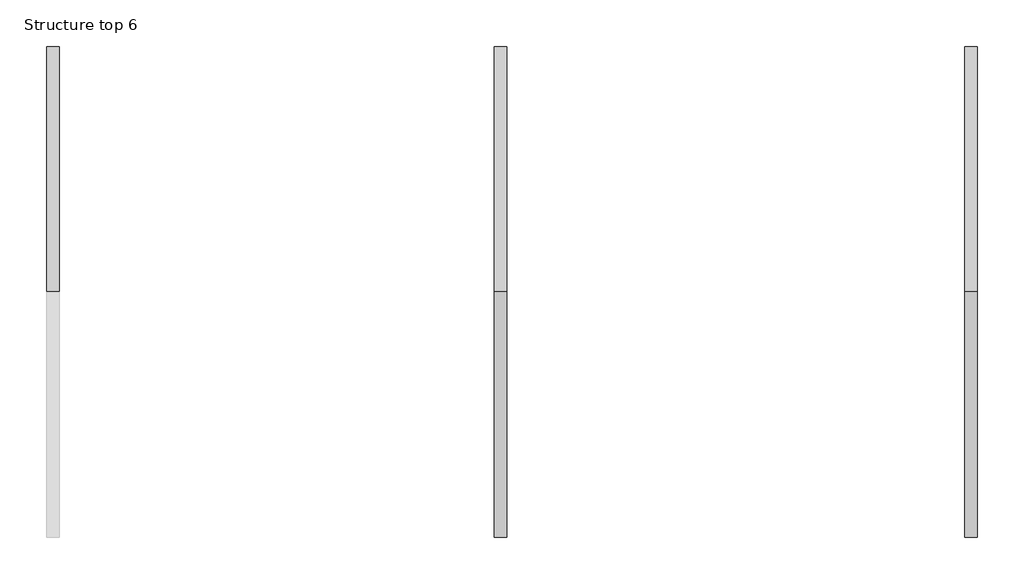
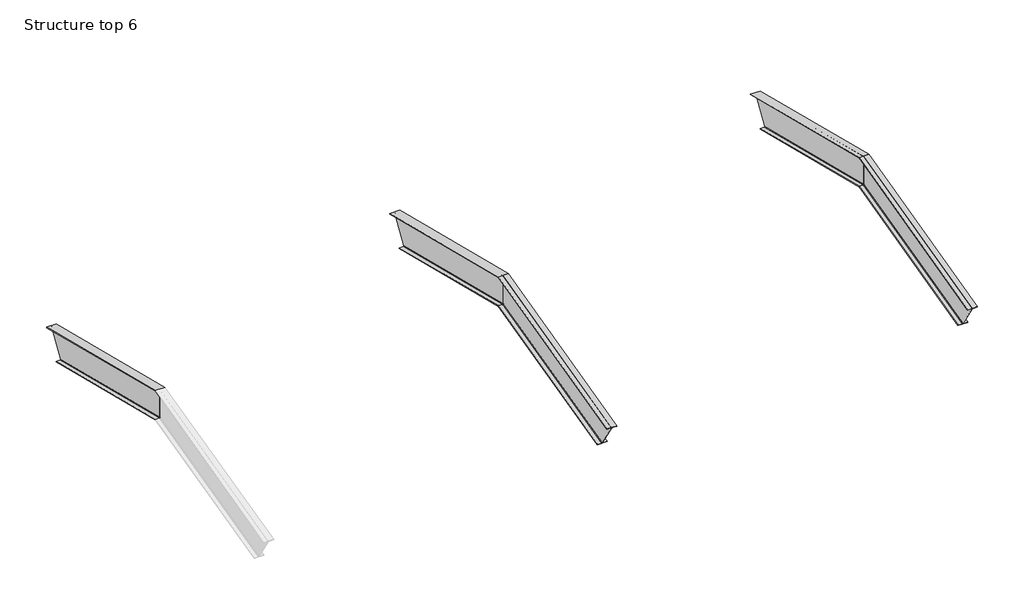
# One storey, part 2 of 2: 5 beams.
"""IFC4 building model written with IfcOpenShell, lengths in millimetres."""

from ifc_helpers import new_model, si_unit, frame, origin, place, context, project, spatial, polyline, ellipse_curve, element, save
from ifc_brep_helpers import plane_surface, revolved_surface, advanced_brep

model = new_model("IFC4")

# Units and contexts
model_context = context("Model", 3, world=origin())
ifc_project = project(units=[si_unit("LENGTHUNIT", "METRE", prefix="MILLI")], contexts=[model_context])

# Site, building, storey
site = spatial("IfcSite", under=ifc_project)
building = spatial("IfcBuilding", under=site)
storey = spatial("IfcBuildingStorey", under=building, Name="Structure top 6", Elevation=5867.6650904)

# Beams
placement = place(None, origin())
element("IfcBeam", 1, ObjectType="W Shapes : W 6X18.5", at=placement, inside=storey, context=model_context, shape_type="AdvancedBrep", body=[
    advanced_brep(
    [(17988.1744333, 7113.772024, 5183.7974927), (18053.8334333, 7113.772024, 5183.7974927), (18053.8334333, 9790.156119, 4514.7014689), (17988.1744333, 9790.156119, 4514.7014689), (17980.5544333, 7113.772024, 5191.6520089), (17980.5544333, 9794.417492, 4521.4906419), (17980.5544333, 7113.772024, 5640.4067021), (17980.5544333, 10037.8839324, 4909.378725), (17988.1744333, 7113.772024, 5648.2612183), (17988.1744333, 10042.1453053, 4916.1678979), (18053.8334333, 7113.772024, 5648.2612183), (18053.8334333, 10042.1453053, 4916.1678979), (18053.8334333, 7113.772024, 5658.2102722), (18053.8334333, 10047.5430444, 4924.7675171), (17901.4334333, 7113.772024, 5658.2102722), (17901.4334333, 10047.5430444, 4924.7675171), (17901.4334333, 7113.772024, 5648.2612183), (17901.4334333, 10042.1453053, 4916.1678979), (17967.0924333, 7113.772024, 5648.2612183), (17967.0924333, 10042.1453053, 4916.1678979), (17974.7124333, 7113.772024, 5640.4067021), (17974.7124333, 10037.8839324, 4909.378725), (17974.7124333, 7113.772024, 5191.6520089), (17974.7124333, 9794.417492, 4521.4906419), (17967.0924333, 7113.772024, 5183.7974927), (17967.0924333, 9790.156119, 4514.7014689), (17901.4334333, 7113.772024, 5183.7974927), (17901.4334333, 9790.156119, 4514.7014689), (17901.4334333, 7113.772024, 5173.8484388), (17901.4334333, 9784.75838, 4506.1018498), (18053.8334333, 7113.772024, 5173.8484388), (18053.8334333, 9784.75838, 4506.1018498)],
    [
        (0, 1),
        (1, 2),
        (2, 3),
        (3, 0),
        (4, 0, ellipse_curve(frame((17988.1744333, 7113.772024, 5191.6520089), z_axis=(0.0, -1.0, 0.0), x_axis=(0.0, 0.0, -1.0)), 7.8545162, 7.62)),
        (3, 5, ellipse_curve(frame((17988.1744333, 9794.417492, 4521.4906419), z_axis=(0.0, 0.8469796531886612, -0.5316253070390979), x_axis=(0.0, 0.5316253070390978, 0.8469796531886611)), 8.0157451, 7.62)),
        (5, 4),
        (6, 4),
        (5, 7),
        (7, 6),
        (8, 6, ellipse_curve(frame((17988.1744333, 7113.772024, 5640.4067021), z_axis=(0.0, -1.0, 0.0), x_axis=(0.0, 0.0, -1.0)), 7.8545162, 7.62)),
        (7, 9, ellipse_curve(frame((17988.1744333, 10037.8839324, 4909.378725), z_axis=(0.0, 0.8469796531886612, -0.5316253070390979), x_axis=(0.0, 0.5316253070390978, 0.8469796531886611)), 8.0157451, 7.62)),
        (9, 8),
        (10, 8),
        (9, 11),
        (11, 10),
        (12, 10),
        (11, 13),
        (13, 12),
        (14, 12),
        (13, 15),
        (15, 14),
        (16, 14),
        (15, 17),
        (17, 16),
        (18, 16),
        (17, 19),
        (19, 18),
        (20, 18, ellipse_curve(frame((17967.0924333, 7113.772024, 5640.4067021), z_axis=(0.0, -1.0, 0.0), x_axis=(0.0, 0.0, -1.0)), 7.8545162, 7.62)),
        (19, 21, ellipse_curve(frame((17967.0924333, 10037.8839324, 4909.378725), z_axis=(0.0, 0.8469796531886612, -0.5316253070390979), x_axis=(0.0, 0.5316253070390978, 0.8469796531886611)), 8.0157451, 7.62)),
        (21, 20),
        (22, 20),
        (21, 23),
        (23, 22),
        (24, 22, ellipse_curve(frame((17967.0924333, 7113.772024, 5191.6520089), z_axis=(0.0, -1.0, 0.0), x_axis=(0.0, 0.0, -1.0)), 7.8545162, 7.62)),
        (23, 25, ellipse_curve(frame((17967.0924333, 9794.417492, 4521.4906419), z_axis=(0.0, 0.8469796531886612, -0.5316253070390979), x_axis=(0.0, 0.5316253070390978, 0.8469796531886611)), 8.0157451, 7.62)),
        (25, 24),
        (26, 24),
        (25, 27),
        (27, 26),
        (28, 26),
        (27, 29),
        (29, 28),
        (30, 28),
        (29, 31),
        (31, 30),
        (1, 30),
        (31, 2),
    ],
    [
        plane_surface(frame((18053.8334333, 7002.1447176, 5211.7043193), z_axis=(0.0, 0.24253562503633308, 0.9701425001453319), x_axis=(0.0, 0.9701425001453319, -0.24253562503633308))),
        revolved_surface(polyline([(17980.5544333, 9796.830743469387, 4520.887328982653), (17980.5544333, 7111.923902529412, 5192.114039217647)]), (17988.1744333, 7003.992839, 5219.0968051), (0.0, 0.9701425001453319, -0.24253562503633308)),
        plane_surface(frame((17980.5544333, 7003.992839, 5219.0968051), z_axis=(1.0, 0.0, 0.0), x_axis=(0.0, 0.9701425001453319, -0.24253562503633308))),
        revolved_surface(polyline([(17980.5544333, 10040.297183869387, 4908.775412082653), (17980.5544333, 7111.923902529412, 5640.868732417647)]), (17988.1744333, 7109.5821786, 5641.4541634), (0.0, 0.9701425001453319, -0.24253562503633308)),
        plane_surface(frame((17988.1744333, 7111.4303001, 5648.8466493), z_axis=(0.0, -0.24253562503633308, -0.9701425001453319), x_axis=(0.0, 0.9701425001453319, -0.24253562503633308))),
        plane_surface(frame((18053.8334333, 7111.4303001, 5648.8466493), z_axis=(1.0, 0.0, 0.0), x_axis=(0.0, 0.9701425001453319, -0.24253562503633308))),
        plane_surface(frame((18053.8334333, 7113.7712539, 5658.2104647), z_axis=(0.0, 0.24253562503633308, 0.9701425001453319), x_axis=(0.0, 0.9701425001453319, -0.24253562503633308))),
        plane_surface(frame((17901.4334333, 7113.7712539, 5658.2104647), z_axis=(-1.0, 0.0, 0.0), x_axis=(0.0, 0.9701425001453319, -0.24253562503633308))),
        plane_surface(frame((17901.4334333, 7111.4303001, 5648.8466493), z_axis=(0.0, -0.24253562503633308, -0.9701425001453319), x_axis=(0.0, 0.9701425001453319, -0.24253562503633308))),
        revolved_surface(polyline([(17959.4724333, 10040.297183869387, 4908.775412082653), (17959.4724333, 7111.923902529412, 5640.868732417647)]), (17967.0924333, 7109.5821786, 5641.4541634), (0.0, 0.9701425001453319, -0.24253562503633308)),
        plane_surface(frame((17974.7124333, 7109.5821786, 5641.4541634), z_axis=(-1.0, 0.0, 0.0), x_axis=(0.0, 0.9701425001453319, -0.24253562503633308))),
        revolved_surface(polyline([(17959.4724333, 9796.830743469387, 4520.887328982653), (17959.4724333, 7111.923902529412, 5192.114039217647)]), (17967.0924333, 7003.992839, 5219.0968051), (0.0, 0.9701425001453319, -0.24253562503633308)),
        plane_surface(frame((17967.0924333, 7002.1447176, 5211.7043193), z_axis=(0.0, 0.24253562503633308, 0.9701425001453319), x_axis=(0.0, 0.9701425001453319, -0.24253562503633308))),
        plane_surface(frame((17901.4334333, 7002.1447176, 5211.7043193), z_axis=(-1.0, 0.0, 0.0), x_axis=(0.0, 0.9701425001453319, -0.24253562503633308))),
        plane_surface(frame((17901.4334333, 6999.8037637, 5202.3405039), z_axis=(0.0, -0.24253562503633308, -0.9701425001453319), x_axis=(0.0, 0.9701425001453319, -0.24253562503633308))),
        plane_surface(frame((18053.8334333, 6999.8037637, 5202.3405039), z_axis=(1.0, 0.0, 0.0), x_axis=(0.0, 0.9701425001453319, -0.24253562503633308))),
        plane_surface(frame((17977.6370052, 7113.772024, 5658.2135449), z_axis=(0.0, -1.0, 0.0), x_axis=(0.0, 0.0, 1.0))),
        plane_surface(frame((17977.6370052, 10047.54482, 4924.7703459), z_axis=(0.0, 0.8469796531886612, -0.5316253070390979), x_axis=(1.0, 0.0, 0.0))),
    ],
    [
        (0, [[1, 2, 3, 4]]),
        (1, [[5, -4, 6, 7]]),
        (2, [[8, -7, 9, 10]]),
        (3, [[11, -10, 12, 13]]),
        (4, [[14, -13, 15, 16]]),
        (5, [[17, -16, 18, 19]]),
        (6, [[20, -19, 21, 22]]),
        (7, [[23, -22, 24, 25]]),
        (8, [[26, -25, 27, 28]]),
        (9, [[29, -28, 30, 31]]),
        (10, [[32, -31, 33, 34]]),
        (11, [[35, -34, 36, 37]]),
        (12, [[38, -37, 39, 40]]),
        (13, [[41, -40, 42, 43]]),
        (14, [[44, -43, 45, 46]]),
        (15, [[47, -46, 48, -2]]),
        (16, [[-1, -5, -8, -11, -14, -17, -20, -23, -26, -29, -32, -35, -38, -41, -44, -47]]),
        (17, [[-48, -45, -42, -39, -36, -33, -30, -27, -24, -21, -18, -15, -12, -9, -6, -3]]),
    ],
),
])
element("IfcBeam", 2, ObjectType="W Shapes : W 6X18.5", at=placement, inside=storey, context=model_context, shape_type="AdvancedBrep", body=[
    advanced_brep(
    [(23341.2244333, 7113.772024, 5183.7974927), (23406.8834333, 7113.772024, 5183.7974927), (23406.8834333, 9790.156119, 4514.7014689), (23341.2244333, 9790.156119, 4514.7014689), (23333.6044333, 7113.772024, 5191.6520089), (23333.6044333, 9794.417492, 4521.4906419), (23333.6044333, 7113.772024, 5640.4067021), (23333.6044333, 10037.8839324, 4909.378725), (23341.2244333, 7113.772024, 5648.2612183), (23341.2244333, 10042.1453053, 4916.1678979), (23406.8834333, 7113.772024, 5648.2612183), (23406.8834333, 10042.1453053, 4916.1678979), (23406.8834333, 7113.772024, 5658.2102722), (23406.8834333, 10047.5430444, 4924.7675171), (23254.4834333, 7113.772024, 5658.2102722), (23254.4834333, 10047.5430444, 4924.7675171), (23254.4834333, 7113.772024, 5648.2612183), (23254.4834333, 10042.1453053, 4916.1678979), (23320.1424333, 7113.772024, 5648.2612183), (23320.1424333, 10042.1453053, 4916.1678979), (23327.7624333, 7113.772024, 5640.4067021), (23327.7624333, 10037.8839324, 4909.378725), (23327.7624333, 7113.772024, 5191.6520089), (23327.7624333, 9794.417492, 4521.4906419), (23320.1424333, 7113.772024, 5183.7974927), (23320.1424333, 9790.156119, 4514.7014689), (23254.4834333, 7113.772024, 5183.7974927), (23254.4834333, 9790.156119, 4514.7014689), (23254.4834333, 7113.772024, 5173.8484388), (23254.4834333, 9784.75838, 4506.1018498), (23406.8834333, 7113.772024, 5173.8484388), (23406.8834333, 9784.75838, 4506.1018498)],
    [
        (0, 1),
        (1, 2),
        (2, 3),
        (3, 0),
        (4, 0, ellipse_curve(frame((23341.2244333, 7113.772024, 5191.6520089), z_axis=(0.0, -1.0, 0.0), x_axis=(0.0, 0.0, -1.0)), 7.8545162, 7.62)),
        (3, 5, ellipse_curve(frame((23341.2244333, 9794.417492, 4521.4906419), z_axis=(0.0, 0.8469796531886612, -0.5316253070390979), x_axis=(0.0, 0.5316253070390978, 0.8469796531886611)), 8.0157451, 7.62)),
        (5, 4),
        (6, 4),
        (5, 7),
        (7, 6),
        (8, 6, ellipse_curve(frame((23341.2244333, 7113.772024, 5640.4067021), z_axis=(0.0, -1.0, 0.0), x_axis=(0.0, 0.0, -1.0)), 7.8545162, 7.62)),
        (7, 9, ellipse_curve(frame((23341.2244333, 10037.8839324, 4909.378725), z_axis=(0.0, 0.8469796531886612, -0.5316253070390979), x_axis=(0.0, 0.5316253070390978, 0.8469796531886611)), 8.0157451, 7.62)),
        (9, 8),
        (10, 8),
        (9, 11),
        (11, 10),
        (12, 10),
        (11, 13),
        (13, 12),
        (14, 12),
        (13, 15),
        (15, 14),
        (16, 14),
        (15, 17),
        (17, 16),
        (18, 16),
        (17, 19),
        (19, 18),
        (20, 18, ellipse_curve(frame((23320.1424333, 7113.772024, 5640.4067021), z_axis=(0.0, -1.0, 0.0), x_axis=(0.0, 0.0, -1.0)), 7.8545162, 7.62)),
        (19, 21, ellipse_curve(frame((23320.1424333, 10037.8839324, 4909.378725), z_axis=(0.0, 0.8469796531886612, -0.5316253070390979), x_axis=(0.0, 0.5316253070390978, 0.8469796531886611)), 8.0157451, 7.62)),
        (21, 20),
        (22, 20),
        (21, 23),
        (23, 22),
        (24, 22, ellipse_curve(frame((23320.1424333, 7113.772024, 5191.6520089), z_axis=(0.0, -1.0, 0.0), x_axis=(0.0, 0.0, -1.0)), 7.8545162, 7.62)),
        (23, 25, ellipse_curve(frame((23320.1424333, 9794.417492, 4521.4906419), z_axis=(0.0, 0.8469796531886612, -0.5316253070390979), x_axis=(0.0, 0.5316253070390978, 0.8469796531886611)), 8.0157451, 7.62)),
        (25, 24),
        (26, 24),
        (25, 27),
        (27, 26),
        (28, 26),
        (27, 29),
        (29, 28),
        (30, 28),
        (29, 31),
        (31, 30),
        (1, 30),
        (31, 2),
    ],
    [
        plane_surface(frame((23406.8834333, 7002.1447176, 5211.7043193), z_axis=(0.0, 0.24253562503633308, 0.9701425001453319), x_axis=(0.0, 0.9701425001453319, -0.24253562503633308))),
        revolved_surface(polyline([(23333.604433300003, 9796.830743469387, 4520.887328982653), (23333.604433300003, 7111.923902529412, 5192.114039217647)]), (23341.2244333, 7003.992839, 5219.0968051), (0.0, 0.9701425001453319, -0.24253562503633308)),
        plane_surface(frame((23333.6044333, 7003.992839, 5219.0968051), z_axis=(1.0, 0.0, 0.0), x_axis=(0.0, 0.9701425001453319, -0.24253562503633308))),
        revolved_surface(polyline([(23333.604433300003, 10040.297183869387, 4908.775412082653), (23333.604433300003, 7111.923902529412, 5640.868732417647)]), (23341.2244333, 7109.5821786, 5641.4541634), (0.0, 0.9701425001453319, -0.24253562503633308)),
        plane_surface(frame((23341.2244333, 7111.4303001, 5648.8466493), z_axis=(0.0, -0.24253562503633308, -0.9701425001453319), x_axis=(0.0, 0.9701425001453319, -0.24253562503633308))),
        plane_surface(frame((23406.8834333, 7111.4303001, 5648.8466493), z_axis=(1.0, 0.0, 0.0), x_axis=(0.0, 0.9701425001453319, -0.24253562503633308))),
        plane_surface(frame((23406.8834333, 7113.7712539, 5658.2104647), z_axis=(0.0, 0.24253562503633308, 0.9701425001453319), x_axis=(0.0, 0.9701425001453319, -0.24253562503633308))),
        plane_surface(frame((23254.4834333, 7113.7712539, 5658.2104647), z_axis=(-1.0, 0.0, 0.0), x_axis=(0.0, 0.9701425001453319, -0.24253562503633308))),
        plane_surface(frame((23254.4834333, 7111.4303001, 5648.8466493), z_axis=(0.0, -0.24253562503633308, -0.9701425001453319), x_axis=(0.0, 0.9701425001453319, -0.24253562503633308))),
        revolved_surface(polyline([(23312.5224333, 10040.297183869387, 4908.775412082653), (23312.5224333, 7111.923902529412, 5640.868732417647)]), (23320.1424333, 7109.5821786, 5641.4541634), (0.0, 0.9701425001453319, -0.24253562503633308)),
        plane_surface(frame((23327.7624333, 7109.5821786, 5641.4541634), z_axis=(-1.0, 0.0, 0.0), x_axis=(0.0, 0.9701425001453319, -0.24253562503633308))),
        revolved_surface(polyline([(23312.5224333, 9796.830743469387, 4520.887328982653), (23312.5224333, 7111.923902529412, 5192.114039217647)]), (23320.1424333, 7003.992839, 5219.0968051), (0.0, 0.9701425001453319, -0.24253562503633308)),
        plane_surface(frame((23320.1424333, 7002.1447176, 5211.7043193), z_axis=(0.0, 0.24253562503633308, 0.9701425001453319), x_axis=(0.0, 0.9701425001453319, -0.24253562503633308))),
        plane_surface(frame((23254.4834333, 7002.1447176, 5211.7043193), z_axis=(-1.0, 0.0, 0.0), x_axis=(0.0, 0.9701425001453319, -0.24253562503633308))),
        plane_surface(frame((23254.4834333, 6999.8037637, 5202.3405039), z_axis=(0.0, -0.24253562503633308, -0.9701425001453319), x_axis=(0.0, 0.9701425001453319, -0.24253562503633308))),
        plane_surface(frame((23406.8834333, 6999.8037637, 5202.3405039), z_axis=(1.0, 0.0, 0.0), x_axis=(0.0, 0.9701425001453319, -0.24253562503633308))),
        plane_surface(frame((23330.6870052, 7113.772024, 5658.2135449), z_axis=(0.0, -1.0, 0.0), x_axis=(0.0, 0.0, 1.0))),
        plane_surface(frame((23330.6870052, 10047.54482, 4924.7703459), z_axis=(0.0, 0.8469796531886612, -0.5316253070390979), x_axis=(1.0, 0.0, 0.0))),
    ],
    [
        (0, [[1, 2, 3, 4]]),
        (1, [[5, -4, 6, 7]]),
        (2, [[8, -7, 9, 10]]),
        (3, [[11, -10, 12, 13]]),
        (4, [[14, -13, 15, 16]]),
        (5, [[17, -16, 18, 19]]),
        (6, [[20, -19, 21, 22]]),
        (7, [[23, -22, 24, 25]]),
        (8, [[26, -25, 27, 28]]),
        (9, [[29, -28, 30, 31]]),
        (10, [[32, -31, 33, 34]]),
        (11, [[35, -34, 36, 37]]),
        (12, [[38, -37, 39, 40]]),
        (13, [[41, -40, 42, 43]]),
        (14, [[44, -43, 45, 46]]),
        (15, [[47, -46, 48, -2]]),
        (16, [[-1, -5, -8, -11, -14, -17, -20, -23, -26, -29, -32, -35, -38, -41, -44, -47]]),
        (17, [[-48, -45, -42, -39, -36, -33, -30, -27, -24, -21, -18, -15, -12, -9, -6, -3]]),
    ],
),
])
element("IfcBeam", 3, ObjectType="W Shapes : W 6X18.5", at=placement, inside=storey, context=model_context, shape_type="AdvancedBrep", body=[
    advanced_brep(
    [(23341.2244333, 4437.3879289, 4514.7014689), (23406.8834333, 4437.3879289, 4514.7014689), (23406.8834333, 7113.772024, 5183.7974927), (23341.2244333, 7113.772024, 5183.7974927), (23333.6044333, 4433.1265559, 4521.4906419), (23333.6044333, 7113.772024, 5191.6520089), (23333.6044333, 4189.6601155, 4909.378725), (23333.6044333, 7113.772024, 5640.4067021), (23341.2244333, 4185.3987426, 4916.1678979), (23341.2244333, 7113.772024, 5648.2612183), (23406.8834333, 4185.3987426, 4916.1678979), (23406.8834333, 7113.772024, 5648.2612183), (23406.8834333, 4180.0010035, 4924.7675171), (23406.8834333, 7113.772024, 5658.2102722), (23254.4834333, 4180.0010035, 4924.7675171), (23254.4834333, 7113.772024, 5658.2102722), (23254.4834333, 4185.3987426, 4916.1678979), (23254.4834333, 7113.772024, 5648.2612183), (23320.1424333, 4185.3987426, 4916.1678979), (23320.1424333, 7113.772024, 5648.2612183), (23327.7624333, 4189.6601155, 4909.378725), (23327.7624333, 7113.772024, 5640.4067021), (23327.7624333, 4433.1265559, 4521.4906419), (23327.7624333, 7113.772024, 5191.6520089), (23320.1424333, 4437.3879289, 4514.7014689), (23320.1424333, 7113.772024, 5183.7974927), (23254.4834333, 4437.3879289, 4514.7014689), (23254.4834333, 7113.772024, 5183.7974927), (23254.4834333, 4442.7856679, 4506.1018498), (23254.4834333, 7113.772024, 5173.8484388), (23406.8834333, 4442.7856679, 4506.1018498), (23406.8834333, 7113.772024, 5173.8484388)],
    [
        (0, 1),
        (1, 2),
        (2, 3),
        (3, 0),
        (4, 0, ellipse_curve(frame((23341.2244333, 4433.1265559, 4521.4906419), z_axis=(0.0, -0.8469796531886659, -0.5316253070390907), x_axis=(0.0, 0.5316253070390901, -0.8469796531886661)), 8.0157451, 7.62)),
        (3, 5, ellipse_curve(frame((23341.2244333, 7113.772024, 5191.6520089), z_axis=(0.0, 1.0, 0.0), x_axis=(0.0, 0.0, 0.9999999999999999)), 7.8545162, 7.62)),
        (5, 4),
        (6, 4),
        (5, 7),
        (7, 6),
        (8, 6, ellipse_curve(frame((23341.2244333, 4189.6601155, 4909.378725), z_axis=(0.0, -0.8469796531886659, -0.5316253070390907), x_axis=(0.0, 0.5316253070390901, -0.8469796531886661)), 8.0157451, 7.62)),
        (7, 9, ellipse_curve(frame((23341.2244333, 7113.772024, 5640.4067021), z_axis=(0.0, 1.0, 0.0), x_axis=(0.0, 0.0, 0.9999999999999999)), 7.8545162, 7.62)),
        (9, 8),
        (10, 8),
        (9, 11),
        (11, 10),
        (12, 10),
        (11, 13),
        (13, 12),
        (14, 12),
        (13, 15),
        (15, 14),
        (16, 14),
        (15, 17),
        (17, 16),
        (18, 16),
        (17, 19),
        (19, 18),
        (20, 18, ellipse_curve(frame((23320.1424333, 4189.6601155, 4909.378725), z_axis=(0.0, -0.8469796531886659, -0.5316253070390907), x_axis=(0.0, 0.5316253070390901, -0.8469796531886661)), 8.0157451, 7.62)),
        (19, 21, ellipse_curve(frame((23320.1424333, 7113.772024, 5640.4067021), z_axis=(0.0, 1.0, 0.0), x_axis=(0.0, 0.0, 0.9999999999999999)), 7.8545162, 7.62)),
        (21, 20),
        (22, 20),
        (21, 23),
        (23, 22),
        (24, 22, ellipse_curve(frame((23320.1424333, 4433.1265559, 4521.4906419), z_axis=(0.0, -0.8469796531886659, -0.5316253070390907), x_axis=(0.0, 0.5316253070390901, -0.8469796531886661)), 8.0157451, 7.62)),
        (23, 25, ellipse_curve(frame((23320.1424333, 7113.772024, 5191.6520089), z_axis=(0.0, 1.0, 0.0), x_axis=(0.0, 0.0, 0.9999999999999999)), 7.8545162, 7.62)),
        (25, 24),
        (26, 24),
        (25, 27),
        (27, 26),
        (28, 26),
        (27, 29),
        (29, 28),
        (30, 28),
        (29, 31),
        (31, 30),
        (1, 30),
        (31, 2),
    ],
    [
        plane_surface(frame((23406.8834333, 4291.6265344, 4478.2611203), z_axis=(0.0, -0.2425356250363261, 0.9701425001453337), x_axis=(0.0, 0.9701425001453337, 0.2425356250363261))),
        revolved_surface(polyline([(23333.604433300003, 7115.620145464711, 5192.114039241156), (23333.604433300003, 4430.713304430615, 4520.887328982652)]), (23341.2244333, 4289.7784129, 4485.6536061), (0.0, 0.9701425001453337, 0.2425356250363261)),
        plane_surface(frame((23333.6044333, 4289.7784129, 4485.6536061), z_axis=(1.0, 0.0, 0.0), x_axis=(0.0, 0.9701425001453337, 0.2425356250363261))),
        revolved_surface(polyline([(23333.604433300003, 7115.620145464711, 5640.868732441156), (23333.604433300003, 4187.246864030613, 4908.775412082654)]), (23341.2244333, 4184.1890733, 4908.0109644), (0.0, 0.9701425001453337, 0.2425356250363261)),
        plane_surface(frame((23341.2244333, 4182.3409519, 4915.4034503), z_axis=(0.0, 0.2425356250363261, -0.9701425001453337), x_axis=(0.0, 0.9701425001453337, 0.2425356250363261))),
        plane_surface(frame((23406.8834333, 4182.3409519, 4915.4034503), z_axis=(1.0, 0.0, 0.0), x_axis=(0.0, 0.9701425001453337, 0.2425356250363261))),
        plane_surface(frame((23406.8834333, 4179.999998, 4924.7672657), z_axis=(0.0, -0.2425356250363261, 0.9701425001453337), x_axis=(0.0, 0.9701425001453337, 0.2425356250363261))),
        plane_surface(frame((23254.4834333, 4179.999998, 4924.7672657), z_axis=(-1.0, 0.0, 0.0), x_axis=(0.0, 0.9701425001453337, 0.2425356250363261))),
        plane_surface(frame((23254.4834333, 4182.3409519, 4915.4034503), z_axis=(0.0, 0.2425356250363261, -0.9701425001453337), x_axis=(0.0, 0.9701425001453337, 0.2425356250363261))),
        revolved_surface(polyline([(23312.5224333, 7115.620145464711, 5640.868732441156), (23312.5224333, 4187.246864030613, 4908.775412082654)]), (23320.1424333, 4184.1890733, 4908.0109644), (0.0, 0.9701425001453337, 0.2425356250363261)),
        plane_surface(frame((23327.7624333, 4184.1890733, 4908.0109644), z_axis=(-1.0, 0.0, 0.0), x_axis=(0.0, 0.9701425001453337, 0.2425356250363261))),
        revolved_surface(polyline([(23312.5224333, 7115.620145464711, 5192.114039241156), (23312.5224333, 4430.713304430615, 4520.887328982652)]), (23320.1424333, 4289.7784129, 4485.6536061), (0.0, 0.9701425001453337, 0.2425356250363261)),
        plane_surface(frame((23320.1424333, 4291.6265344, 4478.2611203), z_axis=(0.0, -0.2425356250363261, 0.9701425001453337), x_axis=(0.0, 0.9701425001453337, 0.2425356250363261))),
        plane_surface(frame((23254.4834333, 4291.6265344, 4478.2611203), z_axis=(-1.0, 0.0, 0.0), x_axis=(0.0, 0.9701425001453337, 0.2425356250363261))),
        plane_surface(frame((23254.4834333, 4293.9674882, 4468.8973049), z_axis=(0.0, 0.2425356250363261, -0.9701425001453337), x_axis=(0.0, 0.9701425001453337, 0.2425356250363261))),
        plane_surface(frame((23406.8834333, 4293.9674882, 4468.8973049), z_axis=(1.0, 0.0, 0.0), x_axis=(0.0, 0.9701425001453337, 0.2425356250363261))),
        plane_surface(frame((23330.6870052, 7113.772024, 5658.2135449), z_axis=(0.0, 1.0, 0.0), x_axis=(0.0, 0.0, -1.0))),
        plane_surface(frame((23330.6870052, 4179.999228, 4924.7703459), z_axis=(0.0, -0.8469796531886659, -0.5316253070390907), x_axis=(1.0, 0.0, 0.0))),
    ],
    [
        (0, [[1, 2, 3, 4]]),
        (1, [[5, -4, 6, 7]]),
        (2, [[8, -7, 9, 10]]),
        (3, [[11, -10, 12, 13]]),
        (4, [[14, -13, 15, 16]]),
        (5, [[17, -16, 18, 19]]),
        (6, [[20, -19, 21, 22]]),
        (7, [[23, -22, 24, 25]]),
        (8, [[26, -25, 27, 28]]),
        (9, [[29, -28, 30, 31]]),
        (10, [[32, -31, 33, 34]]),
        (11, [[35, -34, 36, 37]]),
        (12, [[38, -37, 39, 40]]),
        (13, [[41, -40, 42, 43]]),
        (14, [[44, -43, 45, 46]]),
        (15, [[47, -46, 48, -2]]),
        (16, [[-48, -45, -42, -39, -36, -33, -30, -27, -24, -21, -18, -15, -12, -9, -6, -3]]),
        (17, [[-1, -5, -8, -11, -14, -17, -20, -23, -26, -29, -32, -35, -38, -41, -44, -47]]),
    ],
),
])
element("IfcBeam", 4, ObjectType="W Shapes : W 6X18.5", at=placement, inside=storey, context=model_context, shape_type="AdvancedBrep", body=[
    advanced_brep(
    [(28967.3244333, 7113.772024, 5183.7974927), (29032.9834333, 7113.772024, 5183.7974927), (29032.9834333, 9790.156119, 4514.7014689), (28967.3244333, 9790.156119, 4514.7014689), (28959.7044333, 7113.772024, 5191.6520089), (28959.7044333, 9794.417492, 4521.4906419), (28959.7044333, 7113.772024, 5640.4067021), (28959.7044333, 10037.8839324, 4909.378725), (28967.3244333, 7113.772024, 5648.2612183), (28967.3244333, 10042.1453053, 4916.1678979), (29032.9834333, 7113.772024, 5648.2612183), (29032.9834333, 10042.1453053, 4916.1678979), (29032.9834333, 7113.772024, 5658.2102722), (29032.9834333, 10047.5430444, 4924.7675171), (28880.5834333, 7113.772024, 5658.2102722), (28880.5834333, 10047.5430444, 4924.7675171), (28880.5834333, 7113.772024, 5648.2612183), (28880.5834333, 10042.1453053, 4916.1678979), (28946.2424333, 7113.772024, 5648.2612183), (28946.2424333, 10042.1453053, 4916.1678979), (28953.8624333, 7113.772024, 5640.4067021), (28953.8624333, 10037.8839324, 4909.378725), (28953.8624333, 7113.772024, 5191.6520089), (28953.8624333, 9794.417492, 4521.4906419), (28946.2424333, 7113.772024, 5183.7974927), (28946.2424333, 9790.156119, 4514.7014689), (28880.5834333, 7113.772024, 5183.7974927), (28880.5834333, 9790.156119, 4514.7014689), (28880.5834333, 7113.772024, 5173.8484388), (28880.5834333, 9784.75838, 4506.1018498), (29032.9834333, 7113.772024, 5173.8484388), (29032.9834333, 9784.75838, 4506.1018498)],
    [
        (0, 1),
        (1, 2),
        (2, 3),
        (3, 0),
        (4, 0, ellipse_curve(frame((28967.3244333, 7113.772024, 5191.6520089), z_axis=(0.0, -1.0, 0.0), x_axis=(0.0, 0.0, -1.0)), 7.8545162, 7.62)),
        (3, 5, ellipse_curve(frame((28967.3244333, 9794.417492, 4521.4906419), z_axis=(0.0, 0.8469796531886612, -0.5316253070390979), x_axis=(0.0, 0.5316253070390978, 0.8469796531886611)), 8.0157451, 7.62)),
        (5, 4),
        (6, 4),
        (5, 7),
        (7, 6),
        (8, 6, ellipse_curve(frame((28967.3244333, 7113.772024, 5640.4067021), z_axis=(0.0, -1.0, 0.0), x_axis=(0.0, 0.0, -1.0)), 7.8545162, 7.62)),
        (7, 9, ellipse_curve(frame((28967.3244333, 10037.8839324, 4909.378725), z_axis=(0.0, 0.8469796531886612, -0.5316253070390979), x_axis=(0.0, 0.5316253070390978, 0.8469796531886611)), 8.0157451, 7.62)),
        (9, 8),
        (10, 8),
        (9, 11),
        (11, 10),
        (12, 10),
        (11, 13),
        (13, 12),
        (14, 12),
        (13, 15),
        (15, 14),
        (16, 14),
        (15, 17),
        (17, 16),
        (18, 16),
        (17, 19),
        (19, 18),
        (20, 18, ellipse_curve(frame((28946.2424333, 7113.772024, 5640.4067021), z_axis=(0.0, -1.0, 0.0), x_axis=(0.0, 0.0, -1.0)), 7.8545162, 7.62)),
        (19, 21, ellipse_curve(frame((28946.2424333, 10037.8839324, 4909.378725), z_axis=(0.0, 0.8469796531886612, -0.5316253070390979), x_axis=(0.0, 0.5316253070390978, 0.8469796531886611)), 8.0157451, 7.62)),
        (21, 20),
        (22, 20),
        (21, 23),
        (23, 22),
        (24, 22, ellipse_curve(frame((28946.2424333, 7113.772024, 5191.6520089), z_axis=(0.0, -1.0, 0.0), x_axis=(0.0, 0.0, -1.0)), 7.8545162, 7.62)),
        (23, 25, ellipse_curve(frame((28946.2424333, 9794.417492, 4521.4906419), z_axis=(0.0, 0.8469796531886612, -0.5316253070390979), x_axis=(0.0, 0.5316253070390978, 0.8469796531886611)), 8.0157451, 7.62)),
        (25, 24),
        (26, 24),
        (25, 27),
        (27, 26),
        (28, 26),
        (27, 29),
        (29, 28),
        (30, 28),
        (29, 31),
        (31, 30),
        (1, 30),
        (31, 2),
    ],
    [
        plane_surface(frame((29032.9834333, 7002.1447176, 5211.7043193), z_axis=(0.0, 0.24253562503633308, 0.9701425001453319), x_axis=(0.0, 0.9701425001453319, -0.24253562503633308))),
        revolved_surface(polyline([(28959.7044333, 9796.830743469387, 4520.887328982653), (28959.7044333, 7111.923902529412, 5192.114039217647)]), (28967.3244333, 7003.992839, 5219.0968051), (0.0, 0.9701425001453319, -0.24253562503633308)),
        plane_surface(frame((28959.7044333, 7003.992839, 5219.0968051), z_axis=(1.0, 0.0, 0.0), x_axis=(0.0, 0.9701425001453319, -0.24253562503633308))),
        revolved_surface(polyline([(28959.7044333, 10040.297183869387, 4908.775412082653), (28959.7044333, 7111.923902529412, 5640.868732417647)]), (28967.3244333, 7109.5821786, 5641.4541634), (0.0, 0.9701425001453319, -0.24253562503633308)),
        plane_surface(frame((28967.3244333, 7111.4303001, 5648.8466493), z_axis=(0.0, -0.24253562503633308, -0.9701425001453319), x_axis=(0.0, 0.9701425001453319, -0.24253562503633308))),
        plane_surface(frame((29032.9834333, 7111.4303001, 5648.8466493), z_axis=(1.0, 0.0, 0.0), x_axis=(0.0, 0.9701425001453319, -0.24253562503633308))),
        plane_surface(frame((29032.9834333, 7113.7712539, 5658.2104647), z_axis=(0.0, 0.24253562503633308, 0.9701425001453319), x_axis=(0.0, 0.9701425001453319, -0.24253562503633308))),
        plane_surface(frame((28880.5834333, 7113.7712539, 5658.2104647), z_axis=(-1.0, 0.0, 0.0), x_axis=(0.0, 0.9701425001453319, -0.24253562503633308))),
        plane_surface(frame((28880.5834333, 7111.4303001, 5648.8466493), z_axis=(0.0, -0.24253562503633308, -0.9701425001453319), x_axis=(0.0, 0.9701425001453319, -0.24253562503633308))),
        revolved_surface(polyline([(28938.622433300003, 10040.297183869387, 4908.775412082653), (28938.622433300003, 7111.923902529412, 5640.868732417647)]), (28946.2424333, 7109.5821786, 5641.4541634), (0.0, 0.9701425001453319, -0.24253562503633308)),
        plane_surface(frame((28953.8624333, 7109.5821786, 5641.4541634), z_axis=(-1.0, 0.0, 0.0), x_axis=(0.0, 0.9701425001453319, -0.24253562503633308))),
        revolved_surface(polyline([(28938.622433300003, 9796.830743469387, 4520.887328982653), (28938.622433300003, 7111.923902529412, 5192.114039217647)]), (28946.2424333, 7003.992839, 5219.0968051), (0.0, 0.9701425001453319, -0.24253562503633308)),
        plane_surface(frame((28946.2424333, 7002.1447176, 5211.7043193), z_axis=(0.0, 0.24253562503633308, 0.9701425001453319), x_axis=(0.0, 0.9701425001453319, -0.24253562503633308))),
        plane_surface(frame((28880.5834333, 7002.1447176, 5211.7043193), z_axis=(-1.0, 0.0, 0.0), x_axis=(0.0, 0.9701425001453319, -0.24253562503633308))),
        plane_surface(frame((28880.5834333, 6999.8037637, 5202.3405039), z_axis=(0.0, -0.24253562503633308, -0.9701425001453319), x_axis=(0.0, 0.9701425001453319, -0.24253562503633308))),
        plane_surface(frame((29032.9834333, 6999.8037637, 5202.3405039), z_axis=(1.0, 0.0, 0.0), x_axis=(0.0, 0.9701425001453319, -0.24253562503633308))),
        plane_surface(frame((28956.7870052, 7113.772024, 5658.2135449), z_axis=(0.0, -1.0, 0.0), x_axis=(0.0, 0.0, 1.0))),
        plane_surface(frame((28956.7870052, 10047.54482, 4924.7703459), z_axis=(0.0, 0.8469796531886612, -0.5316253070390979), x_axis=(1.0, 0.0, 0.0))),
    ],
    [
        (0, [[1, 2, 3, 4]]),
        (1, [[5, -4, 6, 7]]),
        (2, [[8, -7, 9, 10]]),
        (3, [[11, -10, 12, 13]]),
        (4, [[14, -13, 15, 16]]),
        (5, [[17, -16, 18, 19]]),
        (6, [[20, -19, 21, 22]]),
        (7, [[23, -22, 24, 25]]),
        (8, [[26, -25, 27, 28]]),
        (9, [[29, -28, 30, 31]]),
        (10, [[32, -31, 33, 34]]),
        (11, [[35, -34, 36, 37]]),
        (12, [[38, -37, 39, 40]]),
        (13, [[41, -40, 42, 43]]),
        (14, [[44, -43, 45, 46]]),
        (15, [[47, -46, 48, -2]]),
        (16, [[-1, -5, -8, -11, -14, -17, -20, -23, -26, -29, -32, -35, -38, -41, -44, -47]]),
        (17, [[-48, -45, -42, -39, -36, -33, -30, -27, -24, -21, -18, -15, -12, -9, -6, -3]]),
    ],
),
])
element("IfcBeam", 5, ObjectType="W Shapes : W 6X18.5", at=placement, inside=storey, context=model_context, shape_type="AdvancedBrep", body=[
    advanced_brep(
    [(28967.3244333, 4437.3879289, 4514.7014689), (29032.9834333, 4437.3879289, 4514.7014689), (29032.9834333, 7113.772024, 5183.7974927), (28967.3244333, 7113.772024, 5183.7974927), (28959.7044333, 4433.1265559, 4521.4906419), (28959.7044333, 7113.772024, 5191.6520089), (28959.7044333, 4189.6601155, 4909.378725), (28959.7044333, 7113.772024, 5640.4067021), (28967.3244333, 4185.3987426, 4916.1678979), (28967.3244333, 7113.772024, 5648.2612183), (29032.9834333, 4185.3987426, 4916.1678979), (29032.9834333, 7113.772024, 5648.2612183), (29032.9834333, 4180.0010035, 4924.7675171), (29032.9834333, 7113.772024, 5658.2102722), (28880.5834333, 4180.0010035, 4924.7675171), (28880.5834333, 7113.772024, 5658.2102722), (28880.5834333, 4185.3987426, 4916.1678979), (28880.5834333, 7113.772024, 5648.2612183), (28946.2424333, 4185.3987426, 4916.1678979), (28946.2424333, 7113.772024, 5648.2612183), (28953.8624333, 4189.6601155, 4909.378725), (28953.8624333, 7113.772024, 5640.4067021), (28953.8624333, 4433.1265559, 4521.4906419), (28953.8624333, 7113.772024, 5191.6520089), (28946.2424333, 4437.3879289, 4514.7014689), (28946.2424333, 7113.772024, 5183.7974927), (28880.5834333, 4437.3879289, 4514.7014689), (28880.5834333, 7113.772024, 5183.7974927), (28880.5834333, 4442.7856679, 4506.1018498), (28880.5834333, 7113.772024, 5173.8484388), (29032.9834333, 4442.7856679, 4506.1018498), (29032.9834333, 7113.772024, 5173.8484388)],
    [
        (0, 1),
        (1, 2),
        (2, 3),
        (3, 0),
        (4, 0, ellipse_curve(frame((28967.3244333, 4433.1265559, 4521.4906419), z_axis=(0.0, -0.8469796531886659, -0.5316253070390907), x_axis=(0.0, 0.5316253070390901, -0.8469796531886661)), 8.0157451, 7.62)),
        (3, 5, ellipse_curve(frame((28967.3244333, 7113.772024, 5191.6520089), z_axis=(0.0, 1.0, 0.0), x_axis=(0.0, 0.0, 0.9999999999999999)), 7.8545162, 7.62)),
        (5, 4),
        (6, 4),
        (5, 7),
        (7, 6),
        (8, 6, ellipse_curve(frame((28967.3244333, 4189.6601155, 4909.378725), z_axis=(0.0, -0.8469796531886659, -0.5316253070390907), x_axis=(0.0, 0.5316253070390901, -0.8469796531886661)), 8.0157451, 7.62)),
        (7, 9, ellipse_curve(frame((28967.3244333, 7113.772024, 5640.4067021), z_axis=(0.0, 1.0, 0.0), x_axis=(0.0, 0.0, 0.9999999999999999)), 7.8545162, 7.62)),
        (9, 8),
        (10, 8),
        (9, 11),
        (11, 10),
        (12, 10),
        (11, 13),
        (13, 12),
        (14, 12),
        (13, 15),
        (15, 14),
        (16, 14),
        (15, 17),
        (17, 16),
        (18, 16),
        (17, 19),
        (19, 18),
        (20, 18, ellipse_curve(frame((28946.2424333, 4189.6601155, 4909.378725), z_axis=(0.0, -0.8469796531886659, -0.5316253070390907), x_axis=(0.0, 0.5316253070390901, -0.8469796531886661)), 8.0157451, 7.62)),
        (19, 21, ellipse_curve(frame((28946.2424333, 7113.772024, 5640.4067021), z_axis=(0.0, 1.0, 0.0), x_axis=(0.0, 0.0, 0.9999999999999999)), 7.8545162, 7.62)),
        (21, 20),
        (22, 20),
        (21, 23),
        (23, 22),
        (24, 22, ellipse_curve(frame((28946.2424333, 4433.1265559, 4521.4906419), z_axis=(0.0, -0.8469796531886659, -0.5316253070390907), x_axis=(0.0, 0.5316253070390901, -0.8469796531886661)), 8.0157451, 7.62)),
        (23, 25, ellipse_curve(frame((28946.2424333, 7113.772024, 5191.6520089), z_axis=(0.0, 1.0, 0.0), x_axis=(0.0, 0.0, 0.9999999999999999)), 7.8545162, 7.62)),
        (25, 24),
        (26, 24),
        (25, 27),
        (27, 26),
        (28, 26),
        (27, 29),
        (29, 28),
        (30, 28),
        (29, 31),
        (31, 30),
        (1, 30),
        (31, 2),
    ],
    [
        plane_surface(frame((29032.9834333, 4291.6265344, 4478.2611203), z_axis=(0.0, -0.2425356250363261, 0.9701425001453337), x_axis=(0.0, 0.9701425001453337, 0.2425356250363261))),
        revolved_surface(polyline([(28959.7044333, 7115.620145464711, 5192.114039241156), (28959.7044333, 4430.713304430615, 4520.887328982652)]), (28967.3244333, 4289.7784129, 4485.6536061), (0.0, 0.9701425001453337, 0.2425356250363261)),
        plane_surface(frame((28959.7044333, 4289.7784129, 4485.6536061), z_axis=(1.0, 0.0, 0.0), x_axis=(0.0, 0.9701425001453337, 0.2425356250363261))),
        revolved_surface(polyline([(28959.7044333, 7115.620145464711, 5640.868732441156), (28959.7044333, 4187.246864030613, 4908.775412082654)]), (28967.3244333, 4184.1890733, 4908.0109644), (0.0, 0.9701425001453337, 0.2425356250363261)),
        plane_surface(frame((28967.3244333, 4182.3409519, 4915.4034503), z_axis=(0.0, 0.2425356250363261, -0.9701425001453337), x_axis=(0.0, 0.9701425001453337, 0.2425356250363261))),
        plane_surface(frame((29032.9834333, 4182.3409519, 4915.4034503), z_axis=(1.0, 0.0, 0.0), x_axis=(0.0, 0.9701425001453337, 0.2425356250363261))),
        plane_surface(frame((29032.9834333, 4179.999998, 4924.7672657), z_axis=(0.0, -0.2425356250363261, 0.9701425001453337), x_axis=(0.0, 0.9701425001453337, 0.2425356250363261))),
        plane_surface(frame((28880.5834333, 4179.999998, 4924.7672657), z_axis=(-1.0, 0.0, 0.0), x_axis=(0.0, 0.9701425001453337, 0.2425356250363261))),
        plane_surface(frame((28880.5834333, 4182.3409519, 4915.4034503), z_axis=(0.0, 0.2425356250363261, -0.9701425001453337), x_axis=(0.0, 0.9701425001453337, 0.2425356250363261))),
        revolved_surface(polyline([(28938.622433300003, 7115.620145464711, 5640.868732441156), (28938.622433300003, 4187.246864030613, 4908.775412082654)]), (28946.2424333, 4184.1890733, 4908.0109644), (0.0, 0.9701425001453337, 0.2425356250363261)),
        plane_surface(frame((28953.8624333, 4184.1890733, 4908.0109644), z_axis=(-1.0, 0.0, 0.0), x_axis=(0.0, 0.9701425001453337, 0.2425356250363261))),
        revolved_surface(polyline([(28938.622433300003, 7115.620145464711, 5192.114039241156), (28938.622433300003, 4430.713304430615, 4520.887328982652)]), (28946.2424333, 4289.7784129, 4485.6536061), (0.0, 0.9701425001453337, 0.2425356250363261)),
        plane_surface(frame((28946.2424333, 4291.6265344, 4478.2611203), z_axis=(0.0, -0.2425356250363261, 0.9701425001453337), x_axis=(0.0, 0.9701425001453337, 0.2425356250363261))),
        plane_surface(frame((28880.5834333, 4291.6265344, 4478.2611203), z_axis=(-1.0, 0.0, 0.0), x_axis=(0.0, 0.9701425001453337, 0.2425356250363261))),
        plane_surface(frame((28880.5834333, 4293.9674882, 4468.8973049), z_axis=(0.0, 0.2425356250363261, -0.9701425001453337), x_axis=(0.0, 0.9701425001453337, 0.2425356250363261))),
        plane_surface(frame((29032.9834333, 4293.9674882, 4468.8973049), z_axis=(1.0, 0.0, 0.0), x_axis=(0.0, 0.9701425001453337, 0.2425356250363261))),
        plane_surface(frame((28956.7870052, 7113.772024, 5658.2135449), z_axis=(0.0, 1.0, 0.0), x_axis=(0.0, 0.0, -1.0))),
        plane_surface(frame((28956.7870052, 4179.999228, 4924.7703459), z_axis=(0.0, -0.8469796531886659, -0.5316253070390907), x_axis=(1.0, 0.0, 0.0))),
    ],
    [
        (0, [[1, 2, 3, 4]]),
        (1, [[5, -4, 6, 7]]),
        (2, [[8, -7, 9, 10]]),
        (3, [[11, -10, 12, 13]]),
        (4, [[14, -13, 15, 16]]),
        (5, [[17, -16, 18, 19]]),
        (6, [[20, -19, 21, 22]]),
        (7, [[23, -22, 24, 25]]),
        (8, [[26, -25, 27, 28]]),
        (9, [[29, -28, 30, 31]]),
        (10, [[32, -31, 33, 34]]),
        (11, [[35, -34, 36, 37]]),
        (12, [[38, -37, 39, 40]]),
        (13, [[41, -40, 42, 43]]),
        (14, [[44, -43, 45, 46]]),
        (15, [[47, -46, 48, -2]]),
        (16, [[-48, -45, -42, -39, -36, -33, -30, -27, -24, -21, -18, -15, -12, -9, -6, -3]]),
        (17, [[-1, -5, -8, -11, -14, -17, -20, -23, -26, -29, -32, -35, -38, -41, -44, -47]]),
    ],
),
])

save(model, "model.ifc")

# Revit data of these elements
# Type "W Shapes : W 6X18.5"
#   Section Name Key = "W12x26"
#   Assembly Code = "B10"
#   Width = 152.4 mm
#   Web Thickness = 5.842 mm
#   Web Fillet = 7.62 mm
#   Warping Constant = 163001.3 cm⁶
#   Torsional Moment of Inertia = 12.4869 cm⁴
#   Section Area = 7.65 in²
#   Plastic Modulus weak axis = 0.00472801 (stored number, unit not read)
#   Plastic Modulus strong axis = 0.0215278 (stored number, unit not read)
#   Perimeter = 15.0571 m²/m
#   Nominal Weight = 379.441 N/m
#   Moment of Inertia weak axis = 720.08 cm⁴
#   Moment of Inertia strong axis = 8491.12 cm⁴
#   Height = 469.9 mm
#   Flange Thickness = 9.652 mm
#   Elastic Modulus weak axis = 0.00309028 (stored number, unit not read)
#   Elastic Modulus strong axis = 0.0193287 (stored number, unit not read)
#   Centroid Vertical = 234.95 mm
#   Centroid Horizontal = 76.2 mm
#   Length [instance default] = 5' - 0"
#   Structural Material [instance default] = Steel ASTM A992
#   Principal Axes Angle = 0
# Elements 1, 2, 3, 4, 5 (IfcBeam, "W Shapes : W 6X18.5")
#   Comments = ""
#   Structural Material = Steel ASTM A992
#   Phase Created = New Construction
#   Materials on its faces: "Steel ASTM A992"
# Materials
#   "Steel ASTM A992": class "Metal", colour RGB 189 187 185, transparency 0, Description = "Structural steel 50ksi", Cost = 0
